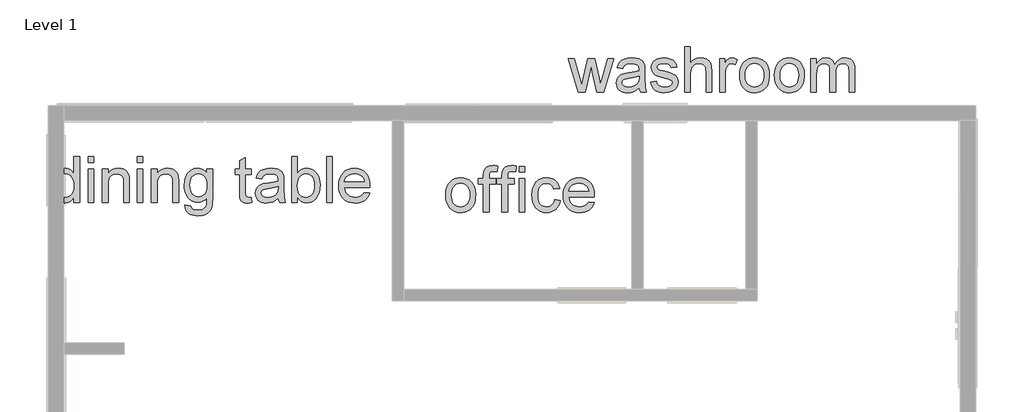
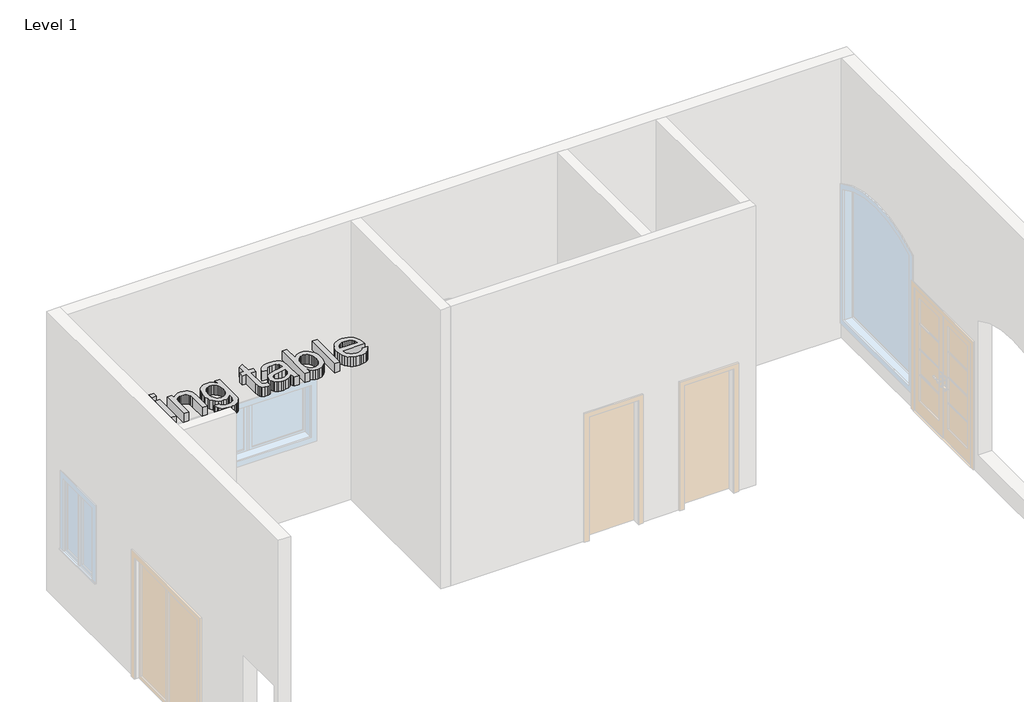
# One storey, part 3 of 3: 3 proxies.
"""IFC4 building model written with IfcOpenShell, lengths in millimetres."""

from ifc_helpers import new_model, si_unit, origin, origin_with_axes, place, context, project, spatial, polyline, outline, extrude, element, save

model = new_model("IFC4")

# Units and contexts
model_context = context("Model", 3, world=origin())
ifc_project = project(units=[si_unit("LENGTHUNIT", "METRE", prefix="MILLI")], contexts=[model_context])

# Site, building, storey
site = spatial("IfcSite", under=ifc_project)
building = spatial("IfcBuilding", under=site)
storey = spatial("IfcBuildingStorey", under=building, Name="Level 1", Elevation=0.0)

# Proxies
placement = place(None, origin())
element("IfcBuildingElementProxy", 1, Name="24\" Arial", ObjectType="24\" Arial", at=placement, inside=storey, context=model_context, shape_type="SweptSolid", body=[
    extrude(outline(polyline([(3479.5195987, 2902.7307881), (3343.4459215, 3350.0637075), (3422.561983, 3350.0637075), (3499.7447573, 3089.0699331), (3522.7954895, 2995.8260034), (3541.6822185, 3085.6495018), (3603.1012663, 3350.0637075), (3693.8170512, 3350.0637075), (3754.9386701, 3086.3930738), (3771.7433975, 3005.0462963), (3795.8351305, 3090.8545059), (3873.1666192, 3350.0637075), (3952.5801096, 3350.0637075), (3815.4654315, 2902.7307881), (3723.411217, 2902.7307881), (3664.9664573, 3165.0629922), (3648.0130155, 3246.8559129), (3572.614814, 2902.7307881), (3479.5195987, 2902.7307881)])), origin_with_axes(), (0.0, 0.0, 1.0), 152.4),
    extrude(outline(polyline([(4290.4592296, 2959.8371182), (4254.0799691, 2928.6442725), (4216.6225293, 2908.2332209), (4177.2318022, 2896.968105), (4135.0526801, 2893.2130664), (4101.1504439, 2895.4716664), (4071.4215056, 2902.2474663), (4045.8658652, 2913.5404661), (4024.4835227, 2929.3506659), (4007.5997908, 2948.6742435), (3995.5399823, 2970.5073765), (3988.3040972, 2994.8500651), (3985.8921355, 3021.7023092), (3989.5356383, 3053.2669409), (4000.4661468, 3081.9316418), (4017.3266421, 3106.469518), (4038.7601052, 3125.6536758), (4063.9486069, 3140.1533299), (4092.0742181, 3150.6376952), (4157.9546979, 3162.0887041), (4235.8066871, 3174.1345707), (4290.0130864, 3188.2624388), (4290.4592296, 3205.2158805), (4285.2170469, 3239.1971213), (4278.6643186, 3251.7820775), (4269.490499, 3261.4299243), (4253.6338259, 3271.0591818), (4234.319543, 3277.9372228), (4185.3181478, 3283.4396557), (4139.9602554, 3279.7775635), (4108.2840879, 3268.7912871), (4086.6833211, 3248.4731821), (4071.5516307, 3216.8156039), (3995.4098572, 3226.3333255), (4008.6268496, 3267.9733579), (4028.3500971, 3300.6905262), (4056.4199404, 3325.7117243), (4094.6767201, 3344.2638459), (4141.4659887, 3355.7520334), (4195.1332983, 3359.5814292), (4246.6070705, 3356.1981766), (4287.4105843, 3346.0484187), (4318.1758761, 3330.7866032), (4339.534982, 3312.067178), (4353.7000288, 3288.9234992), (4362.8831431, 3260.3889235), (4366.6010031, 3193.7648716), (4366.6010031, 3099.0337979), (4370.4675775, 2966.7523379), (4376.193082, 2934.0537589), (4385.6364465, 2902.7307881), (4309.494673, 2902.7307881), (4297.300092, 2929.2019515), (4290.4592296, 2959.8371182)]), holes=[polyline([(4290.4592296, 3112.1206653), (4239.3014755, 3099.4427625), (4167.621134, 3088.7725042), (4102.1124402, 3076.4292089), (4085.0660519, 3067.9896667), (4072.4439171, 3056.3527647), (4064.636411, 3042.4107896), (4062.033909, 3027.0560277), (4067.7036456, 3004.4142601), (4084.7128552, 2985.8621385), (4112.689752, 2973.4816646), (4151.2625499, 2969.3548399), (4192.1590102, 2973.9092185), (4228.2966098, 2987.5723541), (4257.5933469, 3007.7045662), (4277.9672199, 3031.6661741), (4287.0016197, 3056.3527647), (4290.0130864, 3090.5570771), (4290.4592296, 3112.1206653)])]), origin_with_axes(), (0.0, 0.0, 1.0), 152.4),
    extrude(outline(polyline([(4442.7427766, 3035.9788918), (4518.8845501, 3045.4966134), (4523.4854019, 3028.1342071), (4530.893238, 3012.9281595), (4541.1080585, 2999.8784708), (4554.1298633, 2988.9851409), (4569.995831, 2980.3968842), (4588.7431402, 2974.2624152), (4634.8817832, 2969.3548399), (4680.4627472, 2973.8534506), (4698.1783503, 2979.4767139), (4712.5107007, 2987.3492825), (4731.4717869, 3006.9052263), (4736.2120585, 3017.8543241), (4737.792149, 3029.5841725), (4736.2027638, 3039.8640555), (4731.4346083, 3048.9914019), (4712.3619863, 3063.7884848), (4683.8459999, 3073.4549209), (4633.9894968, 3085.5007874), (4564.5026928, 3105.5958209), (4519.3306933, 3122.753745), (4490.3127958, 3141.4731702), (4469.2882973, 3166.2527074), (4456.517448, 3195.5122659), (4452.2604983, 3227.6717552), (4455.6809295, 3257.1729745), (4465.9422232, 3284.4062993), (4482.1149144, 3308.29355), (4503.269538, 3327.7565473), (4524.2940365, 3340.0068961), (4551.6760756, 3350.2867791), (4583.3336538, 3357.2577667), (4617.1847695, 3359.5814292), (4666.7438437, 3355.8449799), (4709.8338415, 3344.6356319), (4744.484297, 3327.0501539), (4768.7247445, 3304.1853147), (4784.7858998, 3274.3494879), (4794.8984791, 3235.8510472), (4718.7567056, 3226.3333255), (4709.1460374, 3250.2949335), (4690.1291833, 3268.3451439), (4661.5202504, 3279.6660277), (4623.1333455, 3283.4396557), (4579.4113115, 3279.8333314), (4550.2632888, 3269.0143587), (4533.8675261, 3253.3993466), (4528.4022718, 3235.404904), (4530.6701664, 3223.6936449), (4537.4738503, 3213.2464582), (4549.1107522, 3203.9146295), (4565.878301, 3196.4417309), (4631.461352, 3180.2318611), (4698.7360293, 3160.3413099), (4743.2202246, 3144.3916904), (4772.7400333, 3127.2523556), (4795.1215507, 3103.7926588), (4809.2308296, 3073.9382427), (4813.9339225, 3037.6147502), (4808.4129004, 3000.0643638), (4791.8498339, 2964.7446935), (4764.8767593, 2934.4255449), (4728.1257129, 2911.8767238), (4683.7344641, 2897.8789808), (4633.8407824, 2893.2130664), (4592.8606702, 2895.4623717), (4557.0669727, 2902.2102877), (4526.4596899, 2913.4568143), (4501.038822, 2929.2019515), (4480.2745737, 2949.3713422), (4463.63715, 2973.8906292), (4451.126551, 3002.7598123), (4442.7427766, 3035.9788918)])), origin_with_axes(), (0.0, 0.0, 1.0), 152.4),
    extrude(outline(polyline([(4899.5934177, 2902.7307881), (4899.5934177, 3511.8649762), (4975.7351912, 3511.8649762), (4975.7351912, 3287.9010877), (5003.7027933, 3319.2612371), (5035.109416, 3341.6613438), (5069.9550592, 3355.1014079), (5108.2397229, 3359.5814292), (5154.2296515, 3354.6924433), (5193.7505037, 3340.0254854), (5224.8689922, 3316.7330923), (5236.5523673, 3302.2845587), (5245.6518298, 3285.9678005), (5257.3630889, 3243.6957319), (5261.2668419, 3185.8830084), (5261.2668419, 2902.7307881), (5185.1250684, 2902.7307881), (5185.1250684, 3178.0011451), (5183.6100404, 3203.7101472), (5179.0649565, 3225.6641107), (5171.4898167, 3243.8630356), (5160.884621, 3258.3069218), (5147.5003248, 3269.3024929), (5131.5878839, 3277.1564722), (5113.1472981, 3281.8688598), (5092.1785675, 3283.4396557), (5060.0004889, 3279.2012952), (5029.7928761, 3266.4862139), (5004.7716781, 3246.5213055), (4988.1528437, 3220.5334639), (4978.8396044, 3185.9945442), (4975.7351912, 3140.3764015), (4975.7351912, 2902.7307881), (4899.5934177, 2902.7307881)])), origin_with_axes(), (0.0, 0.0, 1.0), 152.4),
    extrude(outline(polyline([(5365.9617805, 2902.7307881), (5365.9617805, 3350.0637075), (5432.5858323, 3350.0637075), (5432.5858323, 3283.8857989), (5457.1980658, 3322.2541144), (5479.877012, 3344.8587035), (5502.6303154, 3355.9007478), (5527.4656204, 3359.5814292), (5565.3877928, 3353.7072103), (5603.9048227, 3336.0845538), (5578.4746601, 3267.8246435), (5551.7060679, 3279.5359026), (5524.9374756, 3283.4396557), (5502.2027615, 3279.684617), (5481.8846564, 3268.4195011), (5465.4703043, 3250.4994158), (5454.4468493, 3226.7794687), (5445.1893778, 3184.2471499), (5442.103554, 3137.8482567), (5442.103554, 2902.7307881), (5365.9617805, 2902.7307881)])), origin_with_axes(), (0.0, 0.0, 1.0), 152.4),
    extrude(outline(polyline([(5632.4579878, 3126.3972478), (5636.5755178, 3184.3308018), (5648.9281078, 3234.2523674), (5669.5157577, 3276.1619447), (5698.3384676, 3310.0595335), (5727.3563652, 3331.7253629), (5759.3857294, 3347.2009553), (5794.4265602, 3356.4863107), (5832.4788577, 3359.5814292), (5874.4860288, 3355.8124486), (5912.4686163, 3344.5055068), (5946.4266204, 3325.6606037), (5976.3600411, 3299.2777394), (6000.7910288, 3266.2492003), (6018.2417343, 3227.4672729), (6028.7121577, 3182.931957), (6032.2022988, 3132.6432527), (6030.6593869, 3091.886212), (6026.0306511, 3055.7207285), (6018.3160915, 3024.1468022), (6007.5157081, 2997.164433), (5993.7642733, 2973.8580979), (5977.1965596, 2953.3122739), (5957.8125668, 2935.5269609), (5935.6122951, 2920.5021591), (5911.4601468, 2908.563181), (5886.2205245, 2900.0353396), (5859.8934281, 2894.9186347), (5832.4788577, 2893.2130664), (5789.8582397, 2896.968105), (5751.5224554, 2908.2332209), (5717.4715048, 2927.0084141), (5687.7053879, 2953.2936846), (5663.5346504, 2986.6428891), (5646.2698378, 3026.6098845), (5635.9109503, 3073.1946707), (5632.4579878, 3126.3972478)]), holes=[polyline([(5708.5997613, 3126.5459622), (5710.8025934, 3089.6136701), (5717.4110896, 3057.6354265), (5728.42525, 3030.6112313), (5743.8450745, 3008.5410847), (5762.6016783, 2991.3971026), (5783.6261768, 2979.1514011), (5806.91857, 2971.8039802), (5832.4788577, 2969.3548399), (5857.9090203, 2971.8179222), (5881.108467, 2979.207169), (5902.0771976, 2991.5225804), (5920.8152121, 3008.7641563), (5936.2350366, 3031.0527272), (5947.249197, 3058.5091236), (5953.8576932, 3091.1333454), (5956.0605253, 3128.9253926), (5953.8437512, 3164.6865588), (5947.1934291, 3195.828284), (5936.1095588, 3222.350568), (5920.5921405, 3244.2534109), (5901.7844161, 3261.397393), (5880.8296275, 3273.6430945), (5857.7277747, 3280.9905154), (5832.4788577, 3283.4396557), (5806.91857, 3280.99981), (5783.6261768, 3273.6802731), (5762.6016783, 3261.4810449), (5743.8450745, 3244.4021253), (5728.42525, 3222.3970412), (5717.4110896, 3195.4193194), (5710.8025934, 3163.4689597), (5708.5997613, 3126.5459622)])]), origin_with_axes(), (0.0, 0.0, 1.0), 152.4),
    extrude(outline(polyline([(6098.8263506, 3126.3972478), (6102.9438806, 3184.3308018), (6115.2964706, 3234.2523674), (6135.8841205, 3276.1619447), (6164.7068304, 3310.0595335), (6193.724728, 3331.7253629), (6225.7540922, 3347.2009553), (6260.794923, 3356.4863107), (6298.8472205, 3359.5814292), (6340.8543916, 3355.8124486), (6378.8369791, 3344.5055068), (6412.7949832, 3325.6606037), (6442.7284038, 3299.2777394), (6467.1593916, 3266.2492003), (6484.6100971, 3227.4672729), (6495.0805205, 3182.931957), (6498.5706616, 3132.6432527), (6497.0277497, 3091.886212), (6492.3990139, 3055.7207285), (6484.6844543, 3024.1468022), (6473.8840709, 2997.164433), (6460.1326361, 2973.8580979), (6443.5649224, 2953.3122739), (6424.1809296, 2935.5269609), (6401.9806579, 2920.5021591), (6377.8285096, 2908.563181), (6352.5888873, 2900.0353396), (6326.2617909, 2894.9186347), (6298.8472205, 2893.2130664), (6256.2266025, 2896.968105), (6217.8908182, 2908.2332209), (6183.8398676, 2927.0084141), (6154.0737507, 2953.2936846), (6129.9030132, 2986.6428891), (6112.6382006, 3026.6098845), (6102.2793131, 3073.1946707), (6098.8263506, 3126.3972478)]), holes=[polyline([(6174.9681241, 3126.5459622), (6177.1709562, 3089.6136701), (6183.7794524, 3057.6354265), (6194.7936128, 3030.6112313), (6210.2134373, 3008.5410847), (6228.9700411, 2991.3971026), (6249.9945396, 2979.1514011), (6273.2869327, 2971.8039802), (6298.8472205, 2969.3548399), (6324.2773831, 2971.8179222), (6347.4768297, 2979.207169), (6368.4455603, 2991.5225804), (6387.1835749, 3008.7641563), (6402.6033994, 3031.0527272), (6413.6175598, 3058.5091236), (6420.226056, 3091.1333454), (6422.4288881, 3128.9253926), (6420.212114, 3164.6865588), (6413.5617919, 3195.828284), (6402.4779216, 3222.350568), (6386.9605033, 3244.2534109), (6368.1527789, 3261.397393), (6347.1979902, 3273.6430945), (6324.0961375, 3280.9905154), (6298.8472205, 3283.4396557), (6273.2869327, 3280.99981), (6249.9945396, 3273.6802731), (6228.9700411, 3261.4810449), (6210.2134373, 3244.4021253), (6194.7936128, 3222.3970412), (6183.7794524, 3195.4193194), (6177.1709562, 3163.4689597), (6174.9681241, 3126.5459622)])]), origin_with_axes(), (0.0, 0.0, 1.0), 152.4),
    extrude(outline(polyline([(6584.2301568, 2902.7307881), (6584.2301568, 3350.0637075), (6660.3719303, 3350.0637075), (6660.3719303, 3276.4500788), (6683.2739481, 3310.2640158), (6712.7193996, 3336.7537686), (6747.7044625, 3353.874514), (6787.2253147, 3359.5814292), (6829.5717405, 3353.7629782), (6847.594067, 3346.4899146), (6863.5158026, 3336.3076254), (6877.290474, 3323.5042449), (6888.871608, 3308.3679072), (6905.4532638, 3271.0963604), (6933.207089, 3309.808578), (6964.8646672, 3337.460162), (7000.4259984, 3354.0511124), (7039.8910827, 3359.5814292), (7070.3728876, 3357.2810033), (7097.1275379, 3350.3797256), (7120.1550335, 3338.8775961), (7139.4553744, 3322.7746149), (7154.7125425, 3301.8848888), (7165.6105198, 3276.0225249), (7172.1493061, 3245.1875232), (7174.3289015, 3209.3798838), (7174.3289015, 2902.7307881), (7098.187128, 2902.7307881), (7098.187128, 3176.6627155), (7096.4211445, 3214.6406557), (7091.1231939, 3240.2381221), (7081.1965077, 3257.7678321), (7065.5443169, 3271.5425036), (7045.4121048, 3280.4653677), (7022.0453545, 3283.4396557), (7000.4678243, 3281.5342524), (6980.7956974, 3275.8180426), (6963.0289738, 3266.2910263), (6947.1676534, 3252.9532034), (6934.122612, 3235.4141987), (6924.8047253, 3213.2836368), (6919.2139933, 3186.5615178), (6917.3504159, 3155.2478417), (6917.3504159, 2902.7307881), (6841.2086424, 2902.7307881), (6841.2086424, 3185.1394364), (6836.8029783, 3228.1922556), (6831.2958981, 3245.0899294), (6823.5859858, 3258.9017795), (6813.3665181, 3269.6371003), (6800.3307713, 3277.3051866), (6784.4787456, 3281.9060384), (6765.8104409, 3283.4396557), (6736.4765252, 3279.3500096), (6709.4476828, 3267.0810715), (6687.1405225, 3246.9302701), (6671.9716536, 3219.1950343), (6663.2718611, 3180.7151829), (6660.3719303, 3128.330535), (6660.3719303, 2902.7307881), (6584.2301568, 2902.7307881)])), origin_with_axes(), (0.0, 0.0, 1.0), 152.4),
])
element("IfcBuildingElementProxy", 2, Name="24\" Arial", ObjectType="24\" Arial", at=placement, inside=storey, context=model_context, shape_type="SweptSolid", body=[
    extrude(outline(polyline([(1704.0508855, 1522.3143413), (1708.1684154, 1580.2478953), (1720.5210054, 1630.169461), (1741.1086554, 1672.0790382), (1769.9313653, 1705.9766271), (1798.9492628, 1727.6424564), (1830.978627, 1743.1180488), (1866.0194579, 1752.4034043), (1904.0717553, 1755.4985227), (1946.0789264, 1751.7295421), (1984.061514, 1740.4226003), (2018.0195181, 1721.5776972), (2047.9529387, 1695.194833), (2072.3839264, 1662.1662939), (2089.834632, 1623.3843664), (2100.3050553, 1578.8490505), (2103.7951964, 1528.5603462), (2102.2522845, 1487.8033056), (2097.6235488, 1451.6378221), (2089.9089892, 1420.0638957), (2079.1086058, 1393.0815265), (2065.357171, 1369.7751914), (2048.7894572, 1349.2293674), (2029.4054644, 1331.4440545), (2007.2051927, 1316.4192526), (1983.0530445, 1304.4802746), (1957.8134221, 1295.9524331), (1931.4863258, 1290.8357282), (1904.0717553, 1289.1301599), (1861.4511374, 1292.8851986), (1823.1153531, 1304.1503145), (1789.0644025, 1322.9255077), (1759.2982856, 1349.2107781), (1735.127548, 1382.5599826), (1717.8627355, 1422.526978), (1707.503848, 1469.1117642), (1704.0508855, 1522.3143413)]), holes=[polyline([(1780.192659, 1522.4630557), (1782.395491, 1485.5307636), (1789.0039873, 1453.55252), (1800.0181476, 1426.5283249), (1815.4379721, 1404.4581782), (1834.194576, 1387.3141961), (1855.2190745, 1375.0684947), (1878.5114676, 1367.7210738), (1904.0717553, 1365.2719335), (1929.501918, 1367.7350157), (1952.7013646, 1375.1242626), (1973.6700952, 1387.4396739), (1992.4081098, 1404.6812498), (2007.8279343, 1426.9698207), (2018.8420946, 1454.4262171), (2025.4505908, 1487.0504389), (2027.6534229, 1524.8424862), (2025.4366489, 1560.6036524), (2018.7863267, 1591.7453775), (2007.7024565, 1618.2676615), (1992.1850382, 1640.1705044), (1973.3773137, 1657.3144865), (1952.4225251, 1669.560188), (1929.3206723, 1676.9076089), (1904.0717553, 1679.3567492), (1878.5114676, 1676.9169036), (1855.2190745, 1669.5973666), (1834.194576, 1657.3981384), (1815.4379721, 1640.3192188), (1800.0181476, 1618.3141348), (1789.0039873, 1591.3364129), (1782.395491, 1559.3860532), (1780.192659, 1522.4630557)])]), origin_with_axes(), (0.0, 0.0, 1.0), 152.4),
    extrude(outline(polyline([(2208.490135, 1298.6478816), (2208.490135, 1669.8390275), (2141.8660832, 1669.8390275), (2141.8660832, 1745.980801), (2208.490135, 1745.980801), (2208.490135, 1791.0412647), (2210.4977794, 1828.3314008), (2216.5207127, 1854.5423141), (2231.838296, 1879.8609409), (2255.4838858, 1899.9002065), (2288.5728402, 1912.9498952), (2332.220517, 1917.2997915), (2365.2722927, 1915.2177898), (2401.6701424, 1908.971785), (2390.5165623, 1837.5888723), (2346.6458139, 1841.1580179), (2317.7022735, 1837.9978369), (2298.6854195, 1828.5172938), (2288.1452863, 1810.4113155), (2284.6319085, 1781.3748286), (2284.6319085, 1745.980801), (2370.2914037, 1745.980801), (2370.2914037, 1669.8390275), (2284.6319085, 1669.8390275), (2284.6319085, 1298.6478816), (2208.490135, 1298.6478816)])), origin_with_axes(), (0.0, 0.0, 1.0), 152.4),
    extrude(outline(polyline([(2455.9508989, 1298.6478816), (2455.9508989, 1669.8390275), (2389.3268471, 1669.8390275), (2389.3268471, 1745.980801), (2455.9508989, 1745.980801), (2455.9508989, 1791.0412647), (2457.9585434, 1828.3314008), (2463.9814766, 1854.5423141), (2479.29906, 1879.8609409), (2502.9446498, 1899.9002065), (2536.0336041, 1912.9498952), (2579.6812809, 1917.2997915), (2612.7330566, 1915.2177898), (2649.1309064, 1908.971785), (2637.9773262, 1837.5888723), (2594.1065778, 1841.1580179), (2565.1630375, 1837.9978369), (2546.1461834, 1828.5172938), (2535.6060502, 1810.4113155), (2532.0926724, 1781.3748286), (2532.0926724, 1745.980801), (2617.7521677, 1745.980801), (2617.7521677, 1669.8390275), (2532.0926724, 1669.8390275), (2532.0926724, 1298.6478816), (2455.9508989, 1298.6478816)])), origin_with_axes(), (0.0, 0.0, 1.0), 152.4),
    extrude(outline(polyline([(2684.3762195, 1298.6478816), (2684.3762195, 1745.980801), (2760.517993, 1745.980801), (2760.517993, 1298.6478816), (2684.3762195, 1298.6478816)])), origin_with_axes(), (0.0, 0.0, 1.0), 152.4),
    extrude(outline(polyline([(2684.3762195, 1831.6402963), (2684.3762195, 1907.7820698), (2760.517993, 1907.7820698), (2760.517993, 1831.6402963), (2684.3762195, 1831.6402963)])), origin_with_axes(), (0.0, 0.0, 1.0), 152.4),
    extrude(outline(polyline([(3160.262304, 1460.4491504), (3236.4040775, 1450.9314287), (3228.1225443, 1415.0029588), (3215.1750967, 1383.2106081), (3197.5617348, 1355.5543768), (3175.2824585, 1332.0342647), (3149.2760276, 1313.2637189), (3120.4812016, 1299.8561861), (3088.8979806, 1291.8116665), (3054.5263646, 1289.1301599), (3011.8220947, 1292.8712566), (2973.5327837, 1304.0945466), (2939.6584315, 1322.8000299), (2910.199038, 1348.9877065), (2886.3536132, 1382.16496), (2869.3211669, 1421.8391739), (2859.1016992, 1468.0103482), (2855.6952099, 1520.6784829), (2861.5136609, 1588.4364821), (2868.7867245, 1618.9275817), (2878.9690137, 1647.1600813), (2892.1302382, 1672.5670073), (2908.340108, 1694.5813861), (2927.598623, 1713.2032175), (2949.9057832, 1728.4325017), (2974.2531191, 1740.2738859), (2999.6321612, 1748.7320175), (3026.0429094, 1753.8068964), (3053.4853638, 1755.4985227), (3087.2667695, 1753.1748602), (3117.8229317, 1746.2038726), (3145.1538502, 1734.58556), (3169.2595253, 1718.3199224), (3189.7309921, 1697.7787457), (3206.1592861, 1673.333816), (3218.5444073, 1644.9851332), (3226.8863558, 1612.7326974), (3150.7445823, 1603.2149757), (3136.9327322, 1636.4340551), (3115.4249119, 1660.2469486), (3087.4108366, 1674.5792991), (3054.0802214, 1679.3567492), (3028.2085628, 1677.0052027), (3004.8743438, 1669.9505633), (2984.0775642, 1658.192831), (2965.8182241, 1641.7320057), (2950.9514313, 1620.1870068), (2940.3322936, 1593.1767536), (2933.960811, 1560.7012462), (2931.8369834, 1522.7604845), (2933.9143377, 1484.2481019), (2940.1464006, 1451.3961612), (2950.5331721, 1424.2046623), (2965.0746521, 1402.6736054), (2982.9715009, 1386.3103739), (3003.4243784, 1374.6223514), (3026.4332847, 1367.609538), (3051.9982197, 1365.2719335), (3091.4261254, 1371.1089737), (3108.477161, 1378.405274), (3123.7529184, 1388.6200945), (3136.8258438, 1401.8649709), (3147.2683831, 1418.251439), (3155.0805365, 1437.7794988), (3160.262304, 1460.4491504)])), origin_with_axes(), (0.0, 0.0, 1.0), 152.4),
    extrude(outline(polyline([(3616.2206587, 1431.8959853), (3690.8752882, 1422.3782636), (3679.4289266, 1392.4773743), (3663.9765708, 1366.1270413), (3644.5182209, 1343.3272646), (3621.0538767, 1324.0780443), (3593.8251993, 1308.7883449), (3563.0738495, 1297.867131), (3528.7998273, 1291.3144027), (3491.0031327, 1289.1301599), (3443.7584263, 1292.8991406), (3401.662956, 1304.2060824), (3364.7167219, 1323.0509854), (3332.919724, 1349.4338497), (3307.3501416, 1382.6203978), (3289.0861542, 1421.8763525), (3278.1277617, 1467.2017136), (3274.4749642, 1518.5964813), (3278.1649403, 1571.7339959), (3289.2348686, 1618.5697376), (3307.684749, 1659.1037067), (3333.5145816, 1693.3359029), (3365.2279277, 1720.5320491), (3401.3283486, 1739.9578678), (3441.8158444, 1751.613359), (3486.690415, 1755.4985227), (3530.1196676, 1751.6226536), (3569.3942115, 1739.9950464), (3604.5140469, 1720.615701), (3635.4791736, 1693.4846173), (3660.7559746, 1659.3267783), (3678.8108323, 1618.8671664), (3689.643747, 1572.1057819), (3693.2547186, 1519.0426245), (3692.8085754, 1498.5200371), (3350.6167378, 1498.5200371), (3355.0270492, 1468.135826), (3363.7965516, 1441.5252428), (3376.9252448, 1418.6882875), (3394.413129, 1399.6249602), (3415.2935604, 1384.595511), (3438.5998955, 1373.8601901), (3464.3321343, 1367.4189976), (3492.4902767, 1365.2719335), (3533.0149511, 1369.2500437), (3567.1449062, 1381.1843744), (3594.8801421, 1401.8184976), (3616.2206587, 1431.8959853)]), holes=[polyline([(3350.6167378, 1574.6618106), (3617.1129451, 1574.6618106), (3606.8144728, 1614.8890562), (3597.9566712, 1630.7085507), (3586.6264928, 1643.6652929), (3565.8622445, 1659.280305), (3542.235244, 1670.4338851), (3515.7454912, 1677.1260332), (3486.3929862, 1679.3567492), (3459.6197467, 1677.5768237), (3435.0679285, 1672.2370472), (3412.7375316, 1663.3374198), (3392.6285562, 1650.8779413), (3375.7541189, 1635.4348802), (3363.1273368, 1617.5845047), (3354.7482097, 1597.3268149), (3350.6167378, 1574.6618106)])]), origin_with_axes(), (0.0, 0.0, 1.0), 152.4),
])
element("IfcBuildingElementProxy", 3, Name="24\" Arial", ObjectType="24\" Arial", at=placement, inside=storey, context=model_context, shape_type="SweptSolid", body=[
    extrude(outline(polyline([(-3267.2342998, 1426.2061581), (-3267.2342998, 1498.035214), (-3290.0154871, 1462.4459988), (-3317.6113032, 1437.0251308), (-3350.0217481, 1421.77261), (-3387.2468217, 1416.6884364), (-3412.3795555, 1418.5287771), (-3436.4712886, 1424.0497993), (-3459.5220208, 1433.2515029), (-3481.5317522, 1446.1338879), (-3501.8126787, 1462.3112264), (-3519.6769961, 1481.3977903), (-3535.1247046, 1503.3935798), (-3548.155804, 1528.2985947), (-3558.5007495, 1555.6388079), (-3565.8899964, 1584.9401923), (-3571.8013938, 1649.4264746), (-3566.3547289, 1713.113417), (-3550.014734, 1770.6287118), (-3537.7643852, 1796.254062), (-3522.7999986, 1818.700642), (-3505.1215741, 1837.9684516), (-3484.7291118, 1854.0574909), (-3462.3429471, 1866.7446883), (-3438.6834153, 1875.8069721), (-3413.7505164, 1881.2443424), (-3387.5442505, 1883.0567992), (-3350.2912929, 1877.8703845), (-3317.351053, 1862.3111402), (-3289.4299242, 1838.4610681), (-3267.2342998, 1808.4021697), (-3267.2342998, 2035.3403462), (-3191.0925262, 2035.3403462), (-3191.0925262, 1426.2061581), (-3267.2342998, 1426.2061581)]), holes=[polyline([(-3495.6596203, 1649.7239034), (-3493.5125561, 1612.8009059), (-3487.0713636, 1580.8505463), (-3476.3360428, 1553.8728244), (-3461.3065936, 1531.8677403), (-3443.3586243, 1514.7888208), (-3423.867743, 1502.5895925), (-3402.8339499, 1495.2700556), (-3380.2572448, 1492.8302099), (-3357.5736513, 1495.1585198), (-3336.6653359, 1502.1434493), (-3317.5322987, 1513.7849986), (-3300.1745397, 1530.0831675), (-3285.7631847, 1551.1680812), (-3275.4693597, 1577.1698648), (-3269.2930648, 1608.0885183), (-3267.2342998, 1643.9240418), (-3269.3302434, 1683.2125277), (-3275.6180741, 1716.9056342), (-3286.0977921, 1745.0033615), (-3300.7693973, 1767.5057093), (-3318.508237, 1784.7472852), (-3338.1896585, 1797.0626966), (-3359.813662, 1804.4519434), (-3383.3802473, 1806.9150257), (-3406.4030955, 1804.5495373), (-3427.4368887, 1797.4530719), (-3446.4816267, 1785.6256297), (-3463.5373096, 1769.0672105), (-3477.5908205, 1747.4153232), (-3487.6290426, 1720.3074762), (-3493.6519759, 1687.7436696), (-3495.6596203, 1649.7239034)])]), origin_with_axes(), (0.0, 0.0, 1.0), 152.4),
    extrude(outline(polyline([(-3076.879866, 1426.2061581), (-3076.879866, 1873.5390775), (-3000.7380924, 1873.5390775), (-3000.7380924, 1426.2061581), (-3076.879866, 1426.2061581)])), origin_with_axes(), (0.0, 0.0, 1.0), 152.4),
    extrude(outline(polyline([(-3076.879866, 1959.1985727), (-3076.879866, 2035.3403462), (-3000.7380924, 2035.3403462), (-3000.7380924, 1959.1985727), (-3076.879866, 1959.1985727)])), origin_with_axes(), (0.0, 0.0, 1.0), 152.4),
    extrude(outline(polyline([(-2886.5254322, 1426.2061581), (-2886.5254322, 1873.5390775), (-2810.3836587, 1873.5390775), (-2810.3836587, 1811.0790289), (-2783.9310845, 1842.5693034), (-2752.1619705, 1865.0623566), (-2715.0763167, 1878.5581886), (-2672.674123, 1883.0567992), (-2635.1423259, 1879.4318857), (-2600.7707099, 1868.5571451), (-2572.106009, 1851.7895963), (-2551.6949574, 1830.4862583), (-2537.8459288, 1804.702899), (-2528.8672968, 1774.4952862), (-2524.852008, 1700.8816575), (-2524.852008, 1426.2061581), (-2600.9937815, 1426.2061581), (-2600.9937815, 1690.6203638), (-2603.1873189, 1729.9925016), (-2609.7679312, 1757.9879876), (-2621.9067442, 1778.0458425), (-2640.7748839, 1793.6050868), (-2664.9595634, 1803.587541), (-2693.0479959, 1806.9150257), (-2716.168438, 1805.046801), (-2737.6437271, 1799.442127), (-2757.473863, 1790.1010037), (-2775.6588459, 1777.023431), (-2790.8509515, 1758.722265), (-2801.7024555, 1733.7103616), (-2808.2133579, 1701.9877209), (-2810.3836587, 1663.5543427), (-2810.3836587, 1426.2061581), (-2886.5254322, 1426.2061581)])), origin_with_axes(), (0.0, 0.0, 1.0), 152.4),
    extrude(outline(polyline([(-2420.1570694, 1426.2061581), (-2420.1570694, 1873.5390775), (-2344.0152959, 1873.5390775), (-2344.0152959, 1426.2061581), (-2420.1570694, 1426.2061581)])), origin_with_axes(), (0.0, 0.0, 1.0), 152.4),
    extrude(outline(polyline([(-2420.1570694, 1959.1985727), (-2420.1570694, 2035.3403462), (-2344.0152959, 2035.3403462), (-2344.0152959, 1959.1985727), (-2420.1570694, 1959.1985727)])), origin_with_axes(), (0.0, 0.0, 1.0), 152.4),
    extrude(outline(polyline([(-2229.8026356, 1426.2061581), (-2229.8026356, 1873.5390775), (-2153.6608621, 1873.5390775), (-2153.6608621, 1811.0790289), (-2127.2082879, 1842.5693034), (-2095.4391739, 1865.0623566), (-2058.3535201, 1878.5581886), (-2015.9513264, 1883.0567992), (-1978.4195293, 1879.4318857), (-1944.0479133, 1868.5571451), (-1915.3832124, 1851.7895963), (-1894.9721608, 1830.4862583), (-1881.1231322, 1804.702899), (-1872.1445002, 1774.4952862), (-1868.1292114, 1700.8816575), (-1868.1292114, 1426.2061581), (-1944.2709849, 1426.2061581), (-1944.2709849, 1690.6203638), (-1946.4645223, 1729.9925016), (-1953.0451346, 1757.9879876), (-1965.1839476, 1778.0458425), (-1984.0520873, 1793.6050868), (-2008.2367668, 1803.587541), (-2036.3251994, 1806.9150257), (-2059.4456415, 1805.046801), (-2080.9209305, 1799.442127), (-2100.7510664, 1790.1010037), (-2118.9360493, 1777.023431), (-2134.1281549, 1758.722265), (-2144.9796589, 1733.7103616), (-2151.4905613, 1701.9877209), (-2153.6608621, 1663.5543427), (-2153.6608621, 1426.2061581), (-2229.8026356, 1426.2061581)])), origin_with_axes(), (0.0, 0.0, 1.0), 152.4),
    extrude(outline(polyline([(-1782.4697162, 1388.1352714), (-1706.3279427, 1378.6175497), (-1697.925579, 1354.8232454), (-1681.641352, 1338.4646613), (-1649.6305771, 1325.74958), (-1607.7302945, 1321.5112195), (-1563.0416169, 1326.307259), (-1544.9914064, 1332.3023083), (-1529.8039482, 1340.6953773), (-1506.753216, 1363.7461095), (-1492.6253478, 1394.5299906), (-1488.4985232, 1427.2843375), (-1487.4203438, 1483.3124882), (-1512.7575599, 1458.3284688), (-1541.0318855, 1440.4827406), (-1572.2433205, 1429.7753037), (-1606.3918649, 1426.2061581), (-1648.1387858, 1430.3608667), (-1684.8944796, 1442.8249925), (-1716.6589462, 1463.5985354), (-1743.4321858, 1492.6814955), (-1764.6751086, 1527.573612), (-1779.8486248, 1565.7746238), (-1788.9527346, 1607.2845311), (-1791.9874379, 1652.1033338), (-1786.5407729, 1713.5781495), (-1770.2007781, 1770.1082114), (-1758.089849, 1795.5987892), (-1743.5437216, 1818.0128379), (-1726.5623959, 1837.3503574), (-1707.1458719, 1853.6113477), (-1685.6055203, 1866.4937328), (-1662.2527119, 1875.6954363), (-1637.0874468, 1881.2164585), (-1610.1097249, 1883.0567992), (-1574.5019205, 1878.892796), (-1542.1844221, 1866.4007863), (-1513.1572299, 1845.5807701), (-1487.4203438, 1816.4327474), (-1487.4203438, 1873.5390775), (-1411.2785703, 1873.5390775), (-1411.2785703, 1487.3277771), (-1416.4835743, 1398.1549041), (-1422.9898294, 1364.9869453), (-1432.0985865, 1339.4313049), (-1444.0282699, 1318.8204183), (-1458.9973038, 1300.486721), (-1477.0056884, 1284.430213), (-1498.0534235, 1270.6508942), (-1521.9267322, 1259.5902606), (-1548.4118377, 1251.6898081), (-1577.5087398, 1246.9495365), (-1609.2174385, 1245.369446), (-1646.5215167, 1247.5955147), (-1680.0612615, 1254.2737208), (-1709.8366731, 1265.4040643), (-1735.8477513, 1280.9865451), (-1756.8583079, 1301.0397527), (-1771.6321542, 1325.5822763), (-1780.1692903, 1354.6141158), (-1782.4697162, 1388.1352714)]), holes=[polyline([(-1715.8456643, 1657.3083379), (-1713.8147833, 1619.6603577), (-1707.7221402, 1587.4683371), (-1697.5677349, 1560.7322762), (-1683.3515676, 1539.4521748), (-1666.0681658, 1523.2190684), (-1646.712057, 1511.6239924), (-1625.2832412, 1504.6669468), (-1601.7817185, 1502.3479316), (-1578.512562, 1504.6530049), (-1557.1859874, 1511.5682245), (-1537.8019946, 1523.0935906), (-1520.3605837, 1539.2291032), (-1505.9492287, 1560.3000749), (-1495.6554038, 1586.6318186), (-1489.4791088, 1618.2243343), (-1487.4203438, 1655.0776219), (-1489.539524, 1690.3926449), (-1495.8970647, 1721.0882268), (-1506.4929658, 1747.1643676), (-1521.3272273, 1768.6210673), (-1539.1450715, 1785.3746741), (-1558.6917207, 1797.3415361), (-1579.9671747, 1804.5216533), (-1602.9714337, 1806.9150257), (-1625.5899647, 1804.5588319), (-1646.4518068, 1797.4902505), (-1665.55696, 1785.7092815), (-1682.9054244, 1769.2159249), (-1697.3167794, 1748.084538), (-1707.6106044, 1722.3894778), (-1713.7868994, 1692.1307444), (-1715.8456643, 1657.3083379)])]), origin_with_axes(), (0.0, 0.0, 1.0), 152.4),
    extrude(outline(polyline([(-897.321599, 1489.7072075), (-887.8038773, 1423.9754421), (-917.9557222, 1418.5101878), (-944.7614931, 1416.6884364), (-981.3080572, 1419.8486175), (-1008.5599713, 1429.3291605), (-1027.8184863, 1443.9403505), (-1040.3848532, 1462.4924721), (-1047.3000728, 1494.3545326), (-1049.6051461, 1548.8955393), (-1049.6051461, 1797.397304), (-1106.7114762, 1797.397304), (-1106.7114762, 1873.5390775), (-1049.6051461, 1873.5390775), (-1049.6051461, 1982.2493049), (-973.4633726, 2027.0123398), (-973.4633726, 1873.5390775), (-897.321599, 1873.5390775), (-897.321599, 1797.397304), (-973.4633726, 1797.397304), (-973.4633726, 1551.1262553), (-969.4480837, 1511.8656533), (-956.4355736, 1497.9608568), (-945.4492972, 1494.1128717), (-930.4849105, 1492.8302099), (-897.321599, 1489.7072075)])), origin_with_axes(), (0.0, 0.0, 1.0), 152.4),
    extrude(outline(polyline([(-535.6481748, 1483.3124882), (-572.0274353, 1452.1196426), (-609.4848751, 1431.708591), (-648.8756022, 1420.4434751), (-691.0547243, 1416.6884364), (-724.9569605, 1418.9470364), (-754.6858988, 1425.7228363), (-780.2415392, 1437.0158362), (-801.6238817, 1452.826036), (-818.5076136, 1472.1496135), (-830.5674221, 1493.9827466), (-837.8033072, 1518.3254351), (-840.2152689, 1545.1776792), (-836.5717661, 1576.7423109), (-825.6412576, 1605.4070118), (-808.7807623, 1629.944888), (-787.3472992, 1649.1290458), (-762.1587975, 1663.6286999), (-734.0331863, 1674.1130652), (-668.1527065, 1685.5640742), (-590.3007173, 1697.6099407), (-536.094318, 1711.7378088), (-535.6481748, 1728.6912506), (-540.8903575, 1762.6724913), (-547.4430858, 1775.2574475), (-556.6169054, 1784.9052943), (-572.4735785, 1794.5345518), (-591.7878614, 1801.4125928), (-640.7892566, 1806.9150257), (-686.147149, 1803.2529336), (-717.8233165, 1792.2666572), (-739.4240834, 1771.9485521), (-754.5557737, 1740.2909739), (-830.6975472, 1749.8086956), (-817.4805548, 1791.448728), (-797.7573073, 1824.1658963), (-769.687464, 1849.1870943), (-731.4306843, 1867.7392159), (-684.6414157, 1879.2274034), (-630.9741061, 1883.0567992), (-579.5003339, 1879.6735466), (-538.6968201, 1869.5237887), (-507.9315283, 1854.2619732), (-486.5724224, 1835.542548), (-472.4073756, 1812.3988692), (-463.2242613, 1783.8642935), (-459.5064013, 1717.2402417), (-459.5064013, 1622.509168), (-455.6398269, 1490.2277079), (-449.9143224, 1457.5291289), (-440.4709579, 1426.2061581), (-516.6127315, 1426.2061581), (-528.8073124, 1452.6773216), (-535.6481748, 1483.3124882)]), holes=[polyline([(-535.6481748, 1635.5960353), (-586.8059289, 1622.9181326), (-658.4862704, 1612.2478743), (-723.9949642, 1599.9045789), (-741.0413525, 1591.4650367), (-753.6634873, 1579.8281348), (-761.4709934, 1565.8861596), (-764.0734954, 1550.5313977), (-758.4037588, 1527.8896301), (-741.3945492, 1509.3375085), (-713.4176524, 1496.9570346), (-674.8448545, 1492.8302099), (-633.9483942, 1497.3845885), (-597.8107946, 1511.0477241), (-568.5140575, 1531.1799362), (-548.1401845, 1555.1415441), (-539.1057847, 1579.8281348), (-536.094318, 1614.0324471), (-535.6481748, 1635.5960353)])]), origin_with_axes(), (0.0, 0.0, 1.0), 152.4),
    extrude(outline(polyline([(-278.6696892, 1426.2061581), (-354.8114627, 1426.2061581), (-354.8114627, 2035.3403462), (-278.6696892, 2035.3403462), (-278.6696892, 1809.4431705), (-253.6299019, 1841.6491331), (-225.3555763, 1864.653392), (-193.8467125, 1878.4559474), (-159.1033105, 1883.0567992), (-119.8798871, 1878.9113853), (-82.8128226, 1866.4751435), (-50.0212971, 1846.5288244), (-23.6244908, 1819.8531786), (-2.9345997, 1786.7084564), (12.7361803, 1747.3549079), (22.6070987, 1703.4283916), (25.8974049, 1656.5647659), (22.4909156, 1602.4884917), (12.2714478, 1554.9184725), (-4.7609985, 1513.8547084), (-28.6064233, 1479.2971994), (-57.2292982, 1451.9058656), (-88.5940949, 1432.3406272), (-122.7008134, 1420.6014841), (-159.5494537, 1416.6884364), (-195.4360977, 1421.7354314), (-227.2516849, 1436.8764164), (-254.9962154, 1462.1113914), (-278.6696892, 1497.4403564), (-278.6696892, 1426.2061581)]), holes=[polyline([(-278.6696892, 1652.9956202), (-273.4646852, 1589.4945708), (-266.9584301, 1565.4400164), (-257.849673, 1546.5161088), (-239.3997926, 1523.0285281), (-217.9570348, 1506.2516847), (-193.5213998, 1496.1855786), (-166.0928874, 1492.8302099), (-143.3209946, 1495.3025869), (-122.1477817, 1502.7197176), (-102.5732487, 1515.0816022), (-84.5973954, 1532.3882407), (-69.5679462, 1554.5931598), (-58.8326253, 1581.6498862), (-52.3914328, 1613.5584199), (-50.2443687, 1650.318761), (-52.3031337, 1687.7762009), (-58.4794286, 1719.9914581), (-68.7732536, 1746.9645326), (-83.1846086, 1768.6954245), (-100.5144837, 1785.4165), (-119.563869, 1797.3601254), (-140.3327646, 1804.5263006), (-162.8211705, 1806.9150257), (-185.5930632, 1804.4426488), (-206.7662761, 1797.025518), (-226.3408092, 1784.6636334), (-244.3166625, 1767.3569949), (-259.3461117, 1745.3751475), (-270.0814325, 1718.9876359), (-276.522625, 1688.1944601), (-278.6696892, 1652.9956202)])]), origin_with_axes(), (0.0, 0.0, 1.0), 152.4),
    extrude(outline(polyline([(111.5569001, 1426.2061581), (111.5569001, 2035.3403462), (187.6986736, 2035.3403462), (187.6986736, 1426.2061581), (111.5569001, 1426.2061581)])), origin_with_axes(), (0.0, 0.0, 1.0), 152.4),
    extrude(outline(polyline([(615.1038632, 1559.4542618), (689.7584927, 1549.9365401), (678.3121311, 1520.0356507), (662.8597754, 1493.6853177), (643.4014254, 1470.8855411), (619.9370813, 1451.6363208), (592.7084038, 1436.3466214), (561.957054, 1425.4254075), (527.6830318, 1418.8726792), (489.8863372, 1416.6884364), (442.6416308, 1420.457417), (400.5461606, 1431.7643589), (363.5999265, 1450.6092619), (331.8029285, 1476.9921262), (306.2333461, 1510.1786743), (287.9693587, 1549.434629), (277.0109663, 1594.7599901), (273.3581688, 1646.1547578), (277.0481449, 1699.2922723), (288.1180731, 1746.1280141), (306.5679536, 1786.6619832), (332.3977861, 1820.8941794), (364.1111322, 1848.0903256), (400.2115532, 1867.5161443), (440.699049, 1879.1716355), (485.5736196, 1883.0567992), (529.0028721, 1879.1809301), (568.2774161, 1867.5533229), (603.3972514, 1848.1739774), (634.3623782, 1821.0428938), (659.6391791, 1786.8850548), (677.6940369, 1746.4254429), (688.5269516, 1699.6640583), (692.1379231, 1646.600901), (691.6917799, 1626.0783136), (349.4999423, 1626.0783136), (353.9102538, 1595.6941025), (362.6797561, 1569.0835193), (375.8084494, 1546.246564), (393.2963335, 1527.1832367), (414.1767649, 1512.1537875), (437.4831, 1501.4184666), (463.2153388, 1494.9772741), (491.3734812, 1492.8302099), (531.8981556, 1496.8083202), (566.0281107, 1508.7426509), (593.7633466, 1529.3767741), (615.1038632, 1559.4542618)]), holes=[polyline([(349.4999423, 1702.2200871), (615.9961496, 1702.2200871), (605.6976773, 1742.4473327), (596.8398758, 1758.2668271), (585.5096973, 1771.2235694), (564.745449, 1786.8385815), (541.1184485, 1797.9921616), (514.6286958, 1804.6843097), (485.2761908, 1806.9150257), (458.5029512, 1805.1351002), (433.951133, 1799.7953237), (411.6207362, 1790.8956963), (391.5117607, 1778.4362178), (374.6373235, 1762.9931567), (362.0105413, 1745.1427812), (353.6314143, 1724.8850913), (349.4999423, 1702.2200871)])]), origin_with_axes(), (0.0, 0.0, 1.0), 152.4),
])

save(model, "model.ifc")

# Revit data of these elements
# Elements 1, 2, 3 (IfcBuildingElementProxy, "24\" Arial")
#   Phase Created = New Construction
